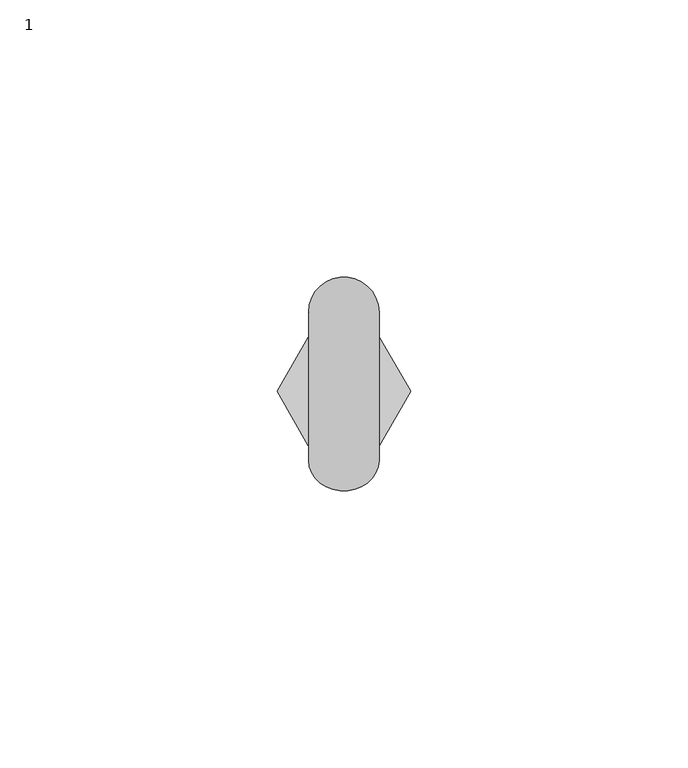
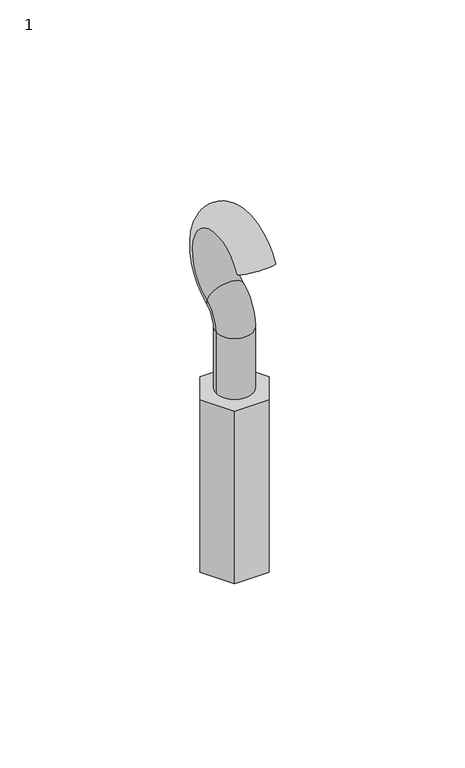
"""IFC4 building model written with IfcOpenShell, lengths in millimetres: proxy geometry, Hanger_Rod-Anvil_International-Weldless_Eye-Fig_248_248L : 1."""

from ifc_helpers import new_model, si_unit, point, frame, origin, origin_with_axes, place, context, project, spatial, polyline, circle_curve, ellipse_curve, trimmed, outline, extrude, source, transform, mapped, element, save
from ifc_brep_helpers import plane_surface, cylinder_surface, revolved_surface, advanced_brep


def proxy_1_89f6120b(model_context):
    return source(origin(), model_context, "Body", "SolidModel", [
        extrude(outline(polyline([(-12.0281557, 0.0), (-6.0140778, 10.4166884), (6.0140778, 10.4166884), (12.0281557, 0.0), (6.0140778, -10.4166884), (-6.0140778, -10.4166884), (-12.0281557, 0.0)])), origin_with_axes(), (0.0, 0.0, 1.0), 63.5),
        advanced_brep(
        [(-6.35, 0.0, 63.5), (6.35, 0.0, 63.5), (6.35, 0.0, 86.1254833), (-6.35, 0.0, 86.1254833), (-6.35, -12.4384419, 114.9797808), (6.35, -12.4384419, 114.9797808), (6.35, 5.715, 94.85529), (-6.35, 5.715, 94.85529)],
        [
            (0, 1, circle_curve(frame((0.0, 0.0, 63.5), z_axis=(0.0, 0.0, -1.0), x_axis=(1.0, 0.0, 0.0)), 6.35)),
            (1, 0, circle_curve(frame((0.0, 0.0, 63.5), z_axis=(0.0, 0.0, -1.0), x_axis=(1.0, 0.0, 0.0)), 6.35)),
            (2, 3, circle_curve(frame((0.0, 0.0, 86.1254833), z_axis=(0.0, 0.0, -1.0), x_axis=(1.0, 0.0, 0.0)), 6.35)),
            (3, 0),
            (1, 2),
            (3, 2, circle_curve(frame((0.0, 0.0, 86.1254833), z_axis=(0.0, 0.0, -1.0), x_axis=(1.0, 0.0, 0.0)), 6.35)),
            (4, 5, circle_curve(frame((0.0, -12.4384419, 114.9797808), z_axis=(0.0, -0.49202315445778766, -0.8705821130010701), x_axis=(1.0, 0.0, 0.0)), 6.35)),
            (5, 4, circle_curve(frame((0.0, -12.4384419, 114.9797808), z_axis=(0.0, -0.49202315445778766, -0.8705821130010701), x_axis=(1.0, 0.0, 0.0)), 6.35)),
            (6, 5, circle_curve(frame((6.35, 0.0, 107.95), z_axis=(1.0, 0.0, 0.0), x_axis=(0.0, -0.8705821130010701, 0.4920231544577876)), 14.2875)),
            (4, 7, circle_curve(frame((-6.35, 0.0, 107.95), z_axis=(-1.0, 0.0, 0.0), x_axis=(0.0, -0.8705821130010701, 0.4920231544577876)), 14.2875)),
            (7, 6, circle_curve(frame((0.0, 5.715, 94.85529), z_axis=(0.0, 0.9165151389911654, 0.4000000000000058), x_axis=(1.0, 0.0, 0.0)), 6.35)),
            (6, 7, circle_curve(frame((0.0, 5.715, 94.85529), z_axis=(0.0, 0.9165151389911657, 0.4000000000000054), x_axis=(1.0, 0.0, 0.0)), 6.35)),
            (2, 6, circle_curve(frame((6.35, 9.525, 86.1254833), z_axis=(-1.0, 0.0, 0.0), x_axis=(0.0, -0.4000000000000002, 0.9165151389911679)), 9.525)),
            (7, 3, circle_curve(frame((-6.35, 9.525, 86.1254833), z_axis=(1.0, 0.0, 0.0), x_axis=(0.0, -0.4000000000000002, 0.9165151389911679)), 9.525)),
        ],
        [
            plane_surface(frame((0.0, -6.35, 63.5), z_axis=(0.0, 0.0, -1.0), x_axis=(1.0, 0.0, 0.0))),
            cylinder_surface(frame((0.0, 0.0, 86.1254833), z_axis=(0.0, 0.0, 1.0), x_axis=(1.0, 0.0, 0.0)), 6.35),
            plane_surface(frame((0.0, -6.9102455, 111.8554338), z_axis=(0.0, -0.49202315445778766, -0.8705821130010701), x_axis=(1.0, 0.0, 0.0))),
            revolved_surface(trimmed(ellipse_curve(frame((0.0, -12.4384419, 114.9797808), z_axis=(0.0, -0.49202315445778766, -0.8705821130010701), x_axis=(1.0, 0.0, 0.0)), 6.35, 6.35), [point((-6.35, -12.4384419, 114.9797808))], [point((6.35, -12.4384419, 114.9797808))], True, "CARTESIAN"), (0.0, 0.0, 107.95), (-1.0, 0.0, 0.0)),
            revolved_surface(trimmed(ellipse_curve(frame((0.0, -12.4384419, 114.9797808), z_axis=(0.0, -0.49202315445778766, -0.8705821130010701), x_axis=(1.0, 0.0, 0.0)), 6.35, 6.35), [point((6.35, -12.4384419, 114.9797808))], [point((-6.35, -12.4384419, 114.9797808))], True, "CARTESIAN"), (0.0, 0.0, 107.95), (-1.0, 0.0, 0.0)),
            revolved_surface(trimmed(ellipse_curve(frame((0.0, 5.715, 94.85529), z_axis=(0.0, 0.9165151389911679, 0.4000000000000001), x_axis=(1.0, 0.0, 0.0)), 6.35, 6.35), [point((-6.35, 5.715, 94.85529))], [point((6.35, 5.715, 94.85529))], True, "CARTESIAN"), (0.0, 9.525, 86.1254833), (1.0, 0.0, 0.0)),
            revolved_surface(trimmed(ellipse_curve(frame((0.0, 5.715, 94.85529), z_axis=(0.0, 0.9165151389911679, 0.4000000000000001), x_axis=(1.0, 0.0, 0.0)), 6.35, 6.35), [point((6.35, 5.715, 94.85529))], [point((-6.35, 5.715, 94.85529))], True, "CARTESIAN"), (0.0, 9.525, 86.1254833), (1.0, 0.0, 0.0)),
        ],
        [
            (0, [[1, 2]]),
            (1, [[3, 4, -2, 5]]),
            (1, [[6, -5, -1, -4]]),
            (2, [[7, 8]]),
            (3, [[9, -7, 10, 11]]),
            (4, [[-10, -8, -9, 12]]),
            (5, [[13, -11, 14, -3]]),
            (6, [[-14, -12, -13, -6]]),
        ],
    ),
    ])


if __name__ == "__main__":
    model = new_model("IFC4")
    model_context = context("Model", 3, world=origin())
    ifc_project = project(units=[si_unit("LENGTHUNIT", "METRE", prefix="MILLI")], contexts=[model_context])
    site = spatial("IfcSite", under=ifc_project)
    building = spatial("IfcBuilding", under=site)
    placement = place(None, origin())
    proxy_1_shape = proxy_1_89f6120b(model_context)
    element("IfcBuildingElementProxy", 1, Name="Hanger_Rod-Anvil_International-Weldless_Eye-Fig_248_248L : 1", ObjectType="Hanger_Rod-Anvil_International-Weldless_Eye-Fig_248_248L : 1", at=placement, inside=building, context=model_context, shape_type="MappedRepresentation", body=[
        mapped(proxy_1_shape, transform((0.0, 0.0, 0.0), x_axis=(1.0, 0.0, 0.0), y_axis=(0.0, 1.0, 0.0), z_axis=(0.0, 0.0, 1.0))),
    ])
    save(model, "model.ifc")

# Revit data of these elements
# Type "Hanger_Rod-Anvil_International-Weldless_Eye-Fig_248_248L : 1"
#   z Error Text [instance default] = "Not Available"
#   URL = "http://www.anvilintl.com/"
#   Product data url = "https://bimobject.com/anvil-international/product/anvil-fig-248"
#   Product Page URL = "http://www.anvilintl.com/products/pipe-hangers-and-hardware/hanger-rods-and-accessories/248-figure-threaded-eye-rod-not-welded---rh"
#   Product Documentation Link = "http://www.anvilintl.com/usercontent/submittal-info-sheet/9579_HG-SUB-FIG248_FIG248L.pdf"
#   Part Number [instance default] = "Contact Anvil Sales for More Options"
#   Part Description [instance default] = "Contact Anvil Sales for More Options"
#   Model Disclaimer = "Contact Anvil International for More Information"
#   Model = "See Part Number"
#   Manufacturer = "Anvil International"
#   Family Version = "1.0"
#   Equipment Number [instance default] = ""
#   Equipment Abbreviation = "HR"
#   Description = "See Part Description"
#   Date Modified = "March 13, 2015"
#   Date Created = "March 13, 2015"
#   Copyright = "Copyright ©2015 Anvil International"
#   z Thread Length [instance default] = 0' - 9"
#   z Overall Width [instance default] = 0' - 2 1/4"
#   z Overall Height [instance default] = 1' - 7"
#   z Overall Depth [instance default] = 0' - 7"
#   z Offset [instance default] = 0' - 0"
#   z Eye to End [instance default] = 1' - 3 1/2"
#   z Eye Radius [instance default] = 0' - 1 1/4"
#   z Eye Diameter [instance default] = 0' - 2 1/2"
#   z Error Box Width [instance default] = 0' - 0.1"
#   z Error Box Height [instance default] = 0' - 0.1"
#   z Error Box Depth [instance default] = 0' - 0.1"
#   z Curve Radius [instance default] = 0' - 2 1/2"
#   z Curve Offset X [instance default] = 0' - 1 3/8"
#   z Curve Offset [instance default] = 0' - 3.48882"
#   z Bolt Radius [instance default] = 0' - 1 1/8"
#   Weight Capacity [instance default] = 10.90 kip
#   Rod Length Actual [instance default] = 0' - 6"
#   Rod Diameter Desired [instance default] = 0' - 2 1/4"
#   Rod Length Desired [instance default] = 0' - 6"
#   Rod Diameter Actual [instance default] = 0' - 2 1/4"
#   Maximum Working Temperature [instance default] = 650 °F
#   Default Elevation = 4' - 0"
#   z Type Thread [instance default] = 1
#   z Type Material = 1
#   z Error [instance default] = no
#   Has Right Hand Threads [instance default] = yes
#   Has Left Hand Threads [instance default] = no
#   Product Material = Carbon Steel - Anvil
# Element 1 (IfcBuildingElementProxy, "Hanger_Rod-Anvil_International-Weldless_Eye-Fig_248_248L : 1")
#   z Thread Length = 0' - 2 1/2"
#   z Overall Width = 0' - 0 1/2"
#   z Overall Height = 0' - 5 1/16"
#   z Overall Depth = 0' - 1 5/8"
#   z Eye to End = 0' - 4 1/4"
#   z Eye Radius = 0' - 0 5/16"
#   z Eye Diameter = 0' - 0 5/8"
#   z Curve Radius = 0' - 0 5/8"
#   z Curve Offset X = 0' - 0 3/8"
#   z Curve Offset = 0' - 0.85923"
#   z Bolt Radius = 0' - 0 1/4"
#   Weight Capacity = 0.24 kip
#   Rod Diameter Desired = 0' - 0 1/2"
#   Rod Diameter Actual = 0' - 0 1/2"
#   Materials on its faces: "THREADED HEX COUPLING (RAW STEEL)", "1/2\" STEEL EYE BOLT (RAW STEEL)"
# Materials
#   "Carbon Steel - Anvil": class "Unassigned", colour RGB 189 187 185, transparency 0
#   "THREADED HEX COUPLING (RAW STEEL)": class "Unassigned", colour RGB 189 187 185, transparency 0, Cost = 0
#   "1/2\" STEEL EYE BOLT (RAW STEEL)": class "Unassigned", colour RGB 189 187 185, transparency 0, Cost = 0
